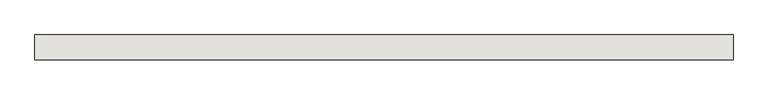
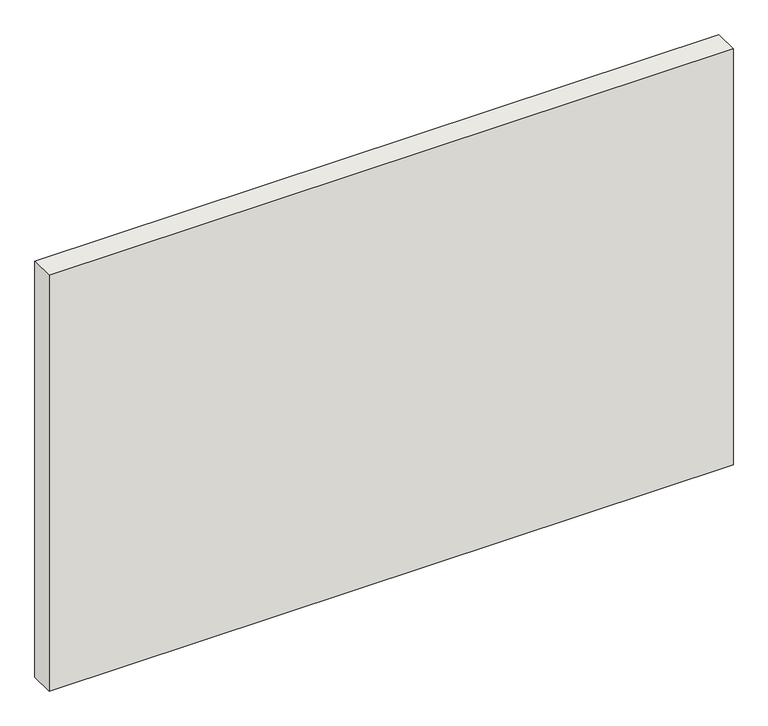
"""IFC4 building model written with IfcOpenShell, lengths in millimetres: wall geometry, Holzwand."""

import ifcopenshell
import ifcopenshell.guid

model = None  # the IFC model being written
_history = None  # IfcOwnerHistory: only IFC2X3 demands one
_inside = {}  # id of a spatial element -> (the spatial element, [elements in it])
_under = {}  # id of a project, library or spatial element -> (it, [spatial elements below it])
_declared = {}  # id of a project -> (the project, [libraries it declares])
_typed = {}  # id of a type object -> (the type object, [elements of that type])
_made_of = {}  # id of a material, layer set ... -> (it, [elements and type objects made of it])


def new_model(schema):
    """Start an empty IFC model of exactly this schema.

    Asked for "IFC4X3", IfcOpenShell would pick the latest addendum, in which some entities
    have other attributes; the version numbers below select the first issue.
    IFC2X3 requires an IfcOwnerHistory on every rooted entity: one is made here for all.
    """
    global model, _history
    if schema == "IFC4X3":
        model = ifcopenshell.file(schema_version=(4, 3, 0, 0))
    else:
        model = ifcopenshell.file(schema=schema)
    _inside.clear()
    _under.clear()
    _declared.clear()
    _typed.clear()
    _made_of.clear()
    _history = None
    if model.schema == "IFC2X3":
        org = make("IfcOrganization", Name="unknown")
        user = make(
            "IfcPersonAndOrganization",
            ThePerson=make("IfcPerson", FamilyName="unknown"),
            TheOrganization=org,
        )
        app = make(
            "IfcApplication",
            ApplicationDeveloper=org,
            Version="unknown",
            ApplicationFullName="unknown",
            ApplicationIdentifier="unknown",
        )
        _history = make(
            "IfcOwnerHistory",
            OwningUser=user,
            OwningApplication=app,
            ChangeAction="ADDED",
            CreationDate=0,
        )
    return model


def make(cls, **values):
    """One entity of the class cls with the attributes given. An attribute that is None is left unset."""
    return model.create_entity(
        cls, **{name: value for name, value in values.items() if value is not None}
    )


def rooted(cls, **values):
    """An entity with a GlobalId (a new one), such as an element, a storey or a relation."""
    return make(cls, GlobalId=ifcopenshell.guid.new(), OwnerHistory=_history, **values)


def si_unit(unit_type, name, prefix=None):
    """IfcSIUnit, for example si_unit("LENGTHUNIT", "METRE", prefix="MILLI")."""
    return make("IfcSIUnit", UnitType=unit_type, Prefix=prefix, Name=name)


def assignment(units):
    """IfcUnitAssignment: the units of a project."""
    return None if units is None else make("IfcUnitAssignment", Units=units)


def point(xyz):
    """IfcCartesianPoint."""
    return None if xyz is None else make("IfcCartesianPoint", Coordinates=xyz)


def direction(xyz):
    """IfcDirection."""
    return None if xyz is None else make("IfcDirection", DirectionRatios=xyz)


def frame(location, z_axis=None, x_axis=None):
    """IfcAxis2Placement3D, a coordinate frame: its origin and axes. An axis left out is left unset."""
    return make(
        "IfcAxis2Placement3D",
        Location=point(location),
        Axis=direction(z_axis),
        RefDirection=direction(x_axis),
    )


def origin():
    """The frame at (0, 0, 0) with its axes left unset."""
    return frame((0.0, 0.0, 0.0))


def origin_with_axes():
    """The frame at (0, 0, 0) with the z axis (0, 0, 1) and the x axis (1, 0, 0) written out."""
    return frame((0.0, 0.0, 0.0), z_axis=(0.0, 0.0, 1.0), x_axis=(1.0, 0.0, 0.0))


def place(relative_to, where):
    """IfcLocalPlacement: puts the frame where relative to a parent placement (None: the world)."""
    return make(
        "IfcLocalPlacement", PlacementRelTo=relative_to, RelativePlacement=where
    )


def context(
    kind, dimensions, precision=None, world=None, true_north=None, identifier=None
):
    """IfcGeometricRepresentationContext, for example the 3D "Model" context."""
    return make(
        "IfcGeometricRepresentationContext",
        ContextIdentifier=identifier,
        ContextType=kind,
        CoordinateSpaceDimension=dimensions,
        Precision=precision,
        WorldCoordinateSystem=world,
        TrueNorth=true_north,
    )


def project(units=None, contexts=None):
    """IfcProject with its units and contexts."""
    return rooted(
        "IfcProject",
        Name="project",
        RepresentationContexts=contexts,
        UnitsInContext=assignment(units),
    )


def spatial(cls, under=None, at=None, **own):
    """A site, building, storey or space (cls), placed at a placement, below another one or the project."""
    s = rooted(cls, ObjectPlacement=at, **own)
    if under is not None:
        _under.setdefault(under.id(), (under, []))[1].append(s)
    return s


def polyline(points):
    """IfcPolyline through the points."""
    return make("IfcPolyline", Points=[point(p) for p in points])


def outline(outer, holes=None, kind="AREA"):
    """IfcArbitraryClosedProfileDef: a profile drawn as a closed curve; with holes, ...WithVoids."""
    if holes is None:
        return make("IfcArbitraryClosedProfileDef", ProfileType=kind, OuterCurve=outer)
    return make(
        "IfcArbitraryProfileDefWithVoids",
        ProfileType=kind,
        OuterCurve=outer,
        InnerCurves=holes,
    )


def extrude(swept, where, along, depth):
    """IfcExtrudedAreaSolid: the profile swept, set in the frame where, extruded along a direction by depth."""
    return make(
        "IfcExtrudedAreaSolid",
        SweptArea=swept,
        Position=where,
        ExtrudedDirection=direction(along),
        Depth=depth,
    )


def shape(context_of_items, identifier, shape_type, items):
    """IfcShapeRepresentation: the items that make up one representation, for example the "Body"."""
    return make(
        "IfcShapeRepresentation",
        ContextOfItems=context_of_items,
        RepresentationIdentifier=identifier,
        RepresentationType=shape_type,
        Items=items,
    )


def source(mapping_origin, context_of_items, identifier, shape_type, items):
    """IfcRepresentationMap: a shape defined once, which mapped items show again and again."""
    return make(
        "IfcRepresentationMap",
        MappingOrigin=mapping_origin,
        MappedRepresentation=shape(context_of_items, identifier, shape_type, items),
    )


def transform(
    local_origin,
    x_axis=None,
    y_axis=None,
    z_axis=None,
    scale=None,
    scale2=None,
    scale3=None,
    uniform=True,
):
    """IfcCartesianTransformationOperator3D, or its non-uniform kind. x_axis, y_axis, z_axis: its Axis1, 2, 3."""
    if uniform:
        return make(
            "IfcCartesianTransformationOperator3D",
            Axis1=direction(x_axis),
            Axis2=direction(y_axis),
            LocalOrigin=point(local_origin),
            Scale=scale,
            Axis3=direction(z_axis),
        )
    return make(
        "IfcCartesianTransformationOperator3DnonUniform",
        Axis1=direction(x_axis),
        Axis2=direction(y_axis),
        LocalOrigin=point(local_origin),
        Scale=scale,
        Axis3=direction(z_axis),
        Scale2=scale2,
        Scale3=scale3,
    )


def mapped(mapping_source, mapping_target):
    """IfcMappedItem: shows the shape of a source again, moved by a transform."""
    return make(
        "IfcMappedItem", MappingSource=mapping_source, MappingTarget=mapping_target
    )


def made_of(thing, what):
    """Note that an element or type object is made of a material, layer set ...; save() writes the relation."""
    if what is not None:
        _made_of.setdefault(what.id(), (what, []))[1].append(thing)
    return thing


def element(
    cls,
    number,
    at=None,
    inside=None,
    cuts=None,
    type_object=None,
    material=None,
    context=None,
    identifier="Body",
    shape_type=None,
    held_by="IfcProductDefinitionShape",
    body=None,
    shapes=None,
    **own,
):
    """One element of the class cls, such as IfcWall. Its Tag is "e" and its number.

    at: its placement. inside: the storey or other place that contains it. cuts: it is an
    opening in that element (IfcRelVoidsElement). A single representation is given by context,
    identifier, shape_type and body (its items); several are given by shapes. held_by: the class
    of the entity that holds the representations. save() writes the other relations.
    """
    e = rooted(cls, Tag="e%d" % number, ObjectPlacement=at, **own)
    if body is not None:
        shapes = [shape(context, identifier, shape_type, body)]
    if shapes is not None:
        e.Representation = make(held_by, Representations=shapes)
    if inside is not None:
        _inside.setdefault(inside.id(), (inside, []))[1].append(e)
    if cuts is not None:
        rooted(
            "IfcRelVoidsElement", RelatingBuildingElement=cuts, RelatedOpeningElement=e
        )
    if type_object is not None:
        _typed.setdefault(type_object.id(), (type_object, []))[1].append(e)
    return made_of(e, material)


def aggregate(whole, parts):
    """IfcRelAggregates: a whole, such as a stair, and the parts it consists of."""
    return rooted("IfcRelAggregates", RelatingObject=whole, RelatedObjects=parts)


def save(model, path):
    """Write the relations noted so far, then the file.

    IfcRelAggregates (storeys below a building ...), IfcRelContainedInSpatialStructure (elements
    in a storey), IfcRelDefinesByType, IfcRelAssociatesMaterial and IfcRelDeclares: one each for
    every whole, place, type object, material and project.
    """
    for whole, parts in _under.values():
        aggregate(whole, parts)
    for where, things in _inside.values():
        rooted(
            "IfcRelContainedInSpatialStructure",
            RelatedElements=things,
            RelatingStructure=where,
        )
    for kind, things in _typed.values():
        rooted("IfcRelDefinesByType", RelatedObjects=things, RelatingType=kind)
    for what, things in _made_of.values():
        rooted("IfcRelAssociatesMaterial", RelatedObjects=things, RelatingMaterial=what)
    for by, libraries in _declared.values():
        rooted("IfcRelDeclares", RelatingContext=by, RelatedDefinitions=libraries)
    model.write(path)


def wall_31205568(model_context):
    return source(origin(), model_context, "Body", "SweptSolid", [
        extrude(outline(polyline([(0.0, 50.0), (1401.2229627, 50.0), (1401.2229627, 0.0), (0.0, 0.0), (0.0, 50.0)])), origin_with_axes(), (0.0, 0.0, 1.0), 900.0),
    ])


if __name__ == "__main__":
    model = new_model("IFC4")
    model_context = context("Model", 3, world=origin())
    ifc_project = project(units=[si_unit("LENGTHUNIT", "METRE", prefix="MILLI")], contexts=[model_context])
    site = spatial("IfcSite", under=ifc_project)
    building = spatial("IfcBuilding", under=site)
    placement = place(None, origin())
    wall_shape = wall_31205568(model_context)
    element("IfcWall", 1, ObjectType="Holzwand", at=placement, inside=building, context=model_context, shape_type="MappedRepresentation", body=[
        mapped(wall_shape, transform((0.0, 0.0, 0.0), x_axis=(1.0, 0.0, 0.0), y_axis=(0.0, 1.0, 0.0), z_axis=(0.0, 0.0, 1.0))),
    ])
    save(model, "model.ifc")

# Revit data of these elements
# Element 1 (IfcWall, "Holzwand")
#   Materials on its faces: "holzschalung"
# Materials
#   "holzschalung": class "Unassigned", colour RGB 128 128 128, transparency 0
